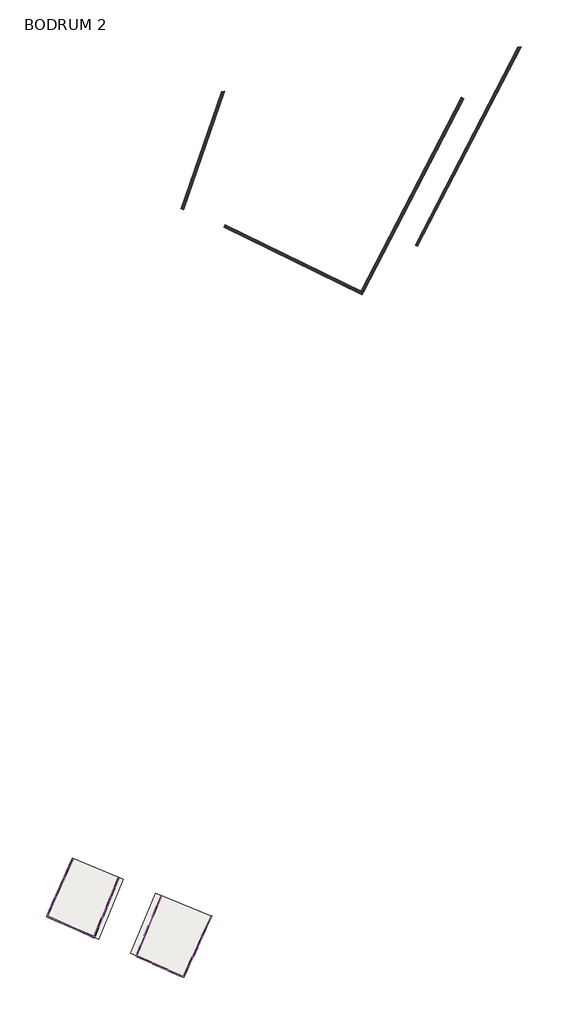
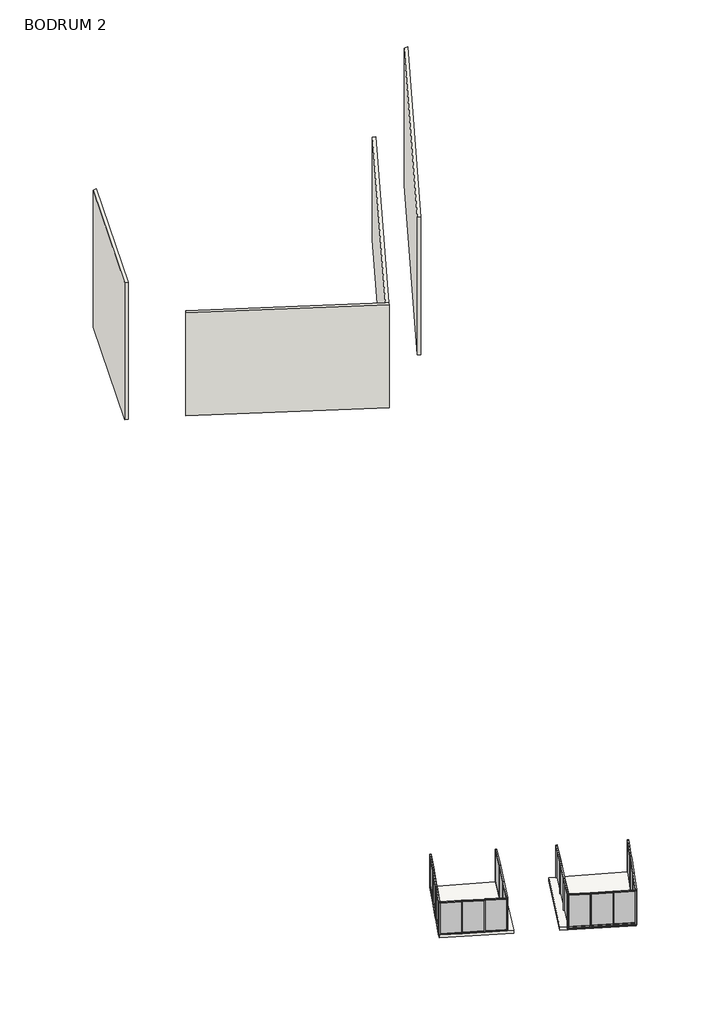
# One storey: 60 members, 18 plates, 4 walls, 1 slab.
# Revit data of these elements (continued)
# Type "Rectangular Mullion : 65 x 125mm rectangular" (continued)
#   built-in parameter 1007300 = 0.106627 (stored number, unit not read)
# Type "System Panel : Glazed"
#   Construction Type Id = "GSP4R"
#   Analytic Construction = "1/8 in Pilkington single glazing"
#   Visual Light Transmittance = 0.9
#   Solar Heat Gain Coefficient = 0.86
#   Heat Transfer Coefficient (U) = 6.7069 W/(m²·K)
#   Define Thermal Properties by = 1
# Type "Generic - 12\""
#   Description = "Generic Floor (Material By Category), 12\" thick"
#   Assembly Code = "B1010"
#   Type Mark = "G01"
#   Function = 0
#   Layers, outside or top first: 30.48 cm no material (function 1)
# Type "Generic - 300mm Masonry"
#   Description = "Generic Wall (Material By Category), 300mm thick, Masonry pattern"
#   Assembly Code = "B2010"
#   Type Mark = "G10"
#   Layers, outside or top first: 30 cm "Gravel" (function 1)
# Elements 1, 2, 3, 4, 5, 6, 7, 8, 9, 10, 11, 12, 13, 14, 15, 16, 17, 18, 19, 20, 21, 22, 23, 24, 25, 26, 27, 28, 29, 30, 31, 32, 33, 34, 35, 36, 37, 38, 39, 40, 41, 42, 43, 44, 45, 46, 47, 48, 49, 50, 51, 52, 53, 54, 55, 56, 57, 58, 59, 60 (IfcMember, "Rectangular Mullion : 65 x 125mm rectangular")
#   Phase Created = New Levels
#   Materials on its faces: "Aluminum"
# Elements 61, 62, 63, 64, 65, 66, 67, 68, 69, 70, 71, 72, 73, 74, 75, 76, 77, 78 (IfcPlate, "System Panel : Glazed")
#   Phase Created = New Levels
#   Materials on its faces: "Glass"
# Element 79 (IfcSlab, "Generic - 12\"")
#   built-in parameter 1001955 = -0.418226 (stored number, unit not read)
#   Height Offset From Level = 20 cm
#   Phase Created = New Levels
#   Materials on its faces: "Default Floor"
# Elements 80, 81 (IfcWall, "Generic - 300mm Masonry")
#   Top Offset = 0 cm
#   Base Offset = 0 cm
#   wall height = 1050 cm
#   Phase Created = New Levels
#   Base Constraint = BODRUM 2
#   Top Constraint = KAT 1
#   Materials on its faces: "Gravel"
# Elements 82, 83 (IfcWall, "Generic - 300mm Masonry")
#   Top Offset = 0 cm
#   Base Offset = 0 cm
#   wall height = 1400 cm
#   Phase Created = New Levels
#   Base Constraint = BODRUM 2
#   Top Constraint = KAT 2
#   Materials on its faces: "Gravel"
# Materials
#   "Gravel": class "Generic", colour RGB 120 120 120, transparency 0, Description = "Crushed stone or gravel", Cost = 0
#   "Aluminum": class "Metal", colour RGB 244 245 246, transparency 0, Description = "Aluminum 6061", Cost = 0
#   "Glass": class "Glass", colour RGB 245 245 243, transparency 1, Description = "Soda Lime Glass", Cost = 0
#   "Default Floor": class "Miscellaneous", colour RGB 128 128 128, transparency 0, Cost = 0
